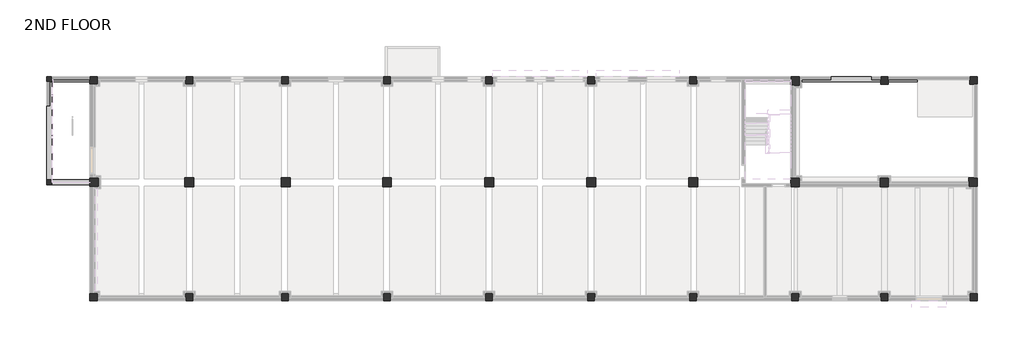
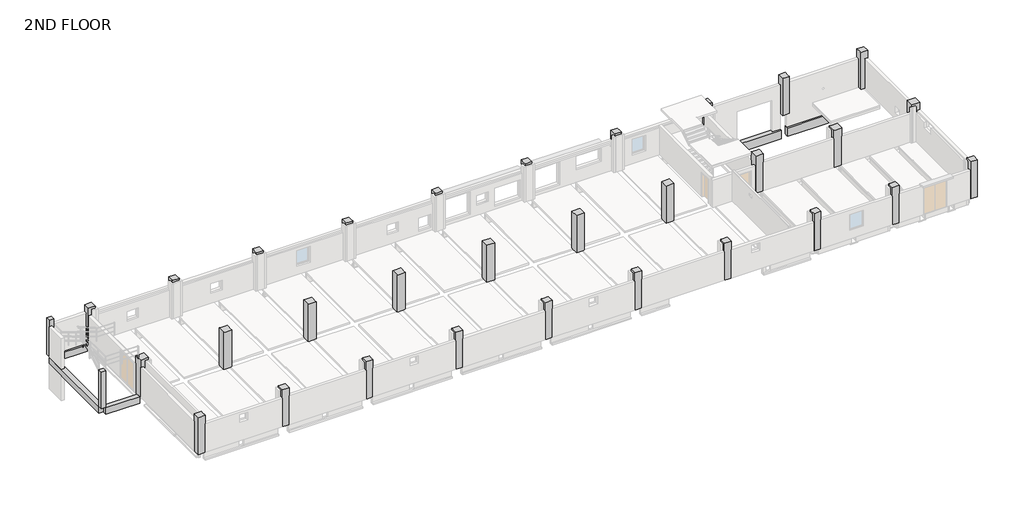
# One storey, part 5 of 7: 32 columns, 8 beams.
"""IFC4 building model written with IfcOpenShell, lengths in millimetres."""

from ifc_helpers import new_model, si_unit, frame, origin, place, context, project, spatial, polyline, outline, extrude, faceted_brep, element, save

model = new_model("IFC4")

# Units and contexts
model_context = context("Model", 3, world=origin())
ifc_project = project(units=[si_unit("LENGTHUNIT", "METRE", prefix="MILLI")], contexts=[model_context])

# Site, building, storey
site = spatial("IfcSite", under=ifc_project)
building = spatial("IfcBuilding", under=site)
storey = spatial("IfcBuildingStorey", under=building, Name="2ND FLOOR", Elevation=10600.0)

# Beams
placement = place(None, origin())
element("IfcBeam", 1, ObjectType="RC Beam_Rectangular : H_SB_AR S16_RC Beam-AG_400x800_2WG1", at=placement, inside=storey, context=model_context, shape_type="Brep", body=[
    faceted_brep([(61700.0, -100.0, 9100.0), (61700.0, 50.0, 9100.0), (61700.0, 300.0, 9100.0), (61000.0, 300.0, 9100.0), (57800.0, 300.0, 9100.0), (55350.0, 300.0, 9100.0), (55350.0, 50.0, 9100.0), (55350.0, -100.0, 9100.0), (61700.0, -100.0, 8300.0), (55350.0, -100.0, 8300.0), (61700.0, 300.0, 8300.0), (61700.0, 50.0, 8300.0), (55350.0, 50.0, 8300.0), (55350.0, 300.0, 8300.0)], [[[0, 1, 2, 3, 4, 5, 6, 7]], [[8, 0, 7, 9]], [[10, 11, 8, 9, 12, 13]], [[2, 10, 13, 5, 4, 3]], [[5, 13, 12, 9, 7, 6]], [[2, 1, 0, 8, 11, 10]]]),
])
element("IfcBeam", 2, ObjectType="RC Beam_Rectangular : H_SB_AR S16_RC Beam-AG_400x800_2WG1", at=placement, inside=storey, context=model_context, shape_type="Brep", body=[
    faceted_brep([(68700.0, -100.0, 9100.0), (68700.0, 50.0, 9100.0), (68700.0, 300.0, 9100.0), (62300.0, 300.0, 9100.0), (62300.0, 50.0, 9100.0), (62300.0, -100.0, 9100.0), (64775.0, -100.0, 9100.0), (64793.0, -100.0, 9100.0), (68700.0, -100.0, 8300.0), (62300.0, -100.0, 8300.0), (64775.0, -100.0, 8300.0), (64793.0, -100.0, 8300.0), (68700.0, 300.0, 8300.0), (68700.0, 50.0, 8300.0), (62300.0, 50.0, 8300.0), (62300.0, 300.0, 8300.0)], [[[0, 1, 2, 3, 4, 5, 6, 7]], [[8, 0, 7, 6, 5, 9, 10, 11]], [[12, 13, 8, 11, 10, 9, 14, 15]], [[2, 12, 15, 3]], [[3, 15, 14, 9, 5, 4]], [[2, 1, 0, 8, 13, 12]]]),
])
element("IfcBeam", 3, ObjectType="RC Beam_Rectangular : H_SB_AR S16_RC Beam-AG_400x600_SWG1", at=placement, inside=storey, context=model_context, shape_type="Brep", body=[
    faceted_brep([(-300.0, -100.0, 10550.0), (-300.0, 50.0, 10550.0), (-300.0, 300.0, 10550.0), (-3300.0, 300.0, 10550.0), (-3300.0, 50.0, 10550.0), (-3300.0, -100.0, 10550.0), (-300.0, -100.0, 9950.0), (-3300.0, -100.0, 9950.0), (-300.0, 300.0, 9950.0), (-300.0, 50.0, 9950.0), (-3300.0, 50.0, 9950.0), (-3300.0, 300.0, 9950.0)], [[[0, 1, 2, 3, 4, 5]], [[6, 0, 5, 7]], [[8, 9, 6, 7, 10, 11]], [[2, 8, 11, 3]], [[2, 1, 0, 6, 9, 8]], [[3, 11, 10, 7, 5, 4]]]),
])
element("IfcBeam", 4, ObjectType="RC Beam_Rectangular : H_SB_AR S16_RC Beam-AG_400x600_SWG2", at=placement, inside=storey, context=model_context, shape_type="Brep", body=[
    faceted_brep([(-3300.0, -100.0, 10550.0), (-3450.0, -100.0, 10550.0), (-3700.0, -100.0, 10550.0), (-3700.0, -2000.0, 10550.0), (-3700.0, -7800.0, 10550.0), (-3300.0, -7800.0, 10550.0), (-3300.0, -100.0, 9950.0), (-3300.0, -7800.0, 9950.0), (-3700.0, -100.0, 9950.0), (-3450.0, -100.0, 9950.0), (-3700.0, -7800.0, 9950.0), (-3700.0, -2000.0, 9950.0)], [[[0, 1, 2, 3, 4, 5]], [[6, 0, 5, 7]], [[8, 9, 6, 7, 10, 11]], [[2, 8, 11, 10, 4, 3]], [[4, 10, 7, 5]], [[2, 1, 0, 6, 9, 8]]]),
])
element("IfcBeam", 5, ObjectType="RC Beam_Rectangular : H_SB_AR S16_RC Beam-AG_400x600_SG1", at=placement, inside=storey, context=model_context, shape_type="SweptSolid", body=[
    extrude(outline(polyline([(-300.0, -7800.0), (-300.0, -8200.0), (-3300.0, -8200.0), (-3300.0, -7800.0), (-300.0, -7800.0)])), frame((0.0, 0.0, 9950.0), z_axis=(0.0, 0.0, 1.0), x_axis=(1.0, 0.0, 0.0)), (0.0, 0.0, 1.0), 600.0),
])
element("IfcBeam", 6, ObjectType="RC Beam_Rectangular : H_SB_AR S16_RC Beam-AG_300x500_2CB1", at=placement, inside=storey, context=model_context, shape_type="Brep", body=[
    faceted_brep([(22850.0, 300.0, 9300.0), (23000.0, 300.0, 9300.0), (23150.0, 300.0, 9300.0), (23150.0, 2350.0, 9300.0), (22850.0, 2350.0, 9300.0), (22850.0, 300.0, 8800.0), (22850.0, 2350.0, 8800.0), (23150.0, 300.0, 8800.0), (23150.0, 2350.0, 8800.0), (23150.0, 300.0, 9150.0), (23150.0, 2350.0, 9150.0)], [[[0, 1, 2, 3, 4]], [[5, 0, 4, 6]], [[7, 5, 6, 8]], [[2, 9, 7, 8, 10, 3]], [[2, 1, 0, 5, 7, 9]], [[3, 10, 8, 6, 4]]]),
])
element("IfcBeam", 7, ObjectType="RC Beam_Rectangular : H_SB_AR S16_RC Beam-AG_300x500_2CB1", at=placement, inside=storey, context=model_context, shape_type="Brep", body=[
    faceted_brep([(27150.0, 2350.0, 9300.0), (26850.0, 2350.0, 9300.0), (26850.0, 300.0, 9300.0), (27000.0, 300.0, 9300.0), (27150.0, 300.0, 9300.0), (26850.0, 2350.0, 9150.0), (26850.0, 2350.0, 8800.0), (26850.0, 300.0, 8800.0), (26850.0, 300.0, 9150.0), (27150.0, 2350.0, 8800.0), (27150.0, 300.0, 8800.0)], [[[0, 1, 2, 3, 4]], [[1, 5, 6, 7, 8, 2]], [[6, 9, 10, 7]], [[9, 0, 4, 10]], [[4, 3, 2, 8, 7, 10]], [[0, 9, 6, 5, 1]]]),
])
element("IfcBeam", 8, ObjectType="RC Beam_Rectangular : H_SB_AR S16_RC Beam-AG_300x500_2CB2", at=placement, inside=storey, context=model_context, shape_type="Brep", body=[
    faceted_brep([(26850.0, 2350.0, 9300.0), (26850.0, 2650.0, 9300.0), (23150.0, 2650.0, 9300.0), (23150.0, 2350.0, 9300.0), (26850.0, 2350.0, 8800.0), (26850.0, 2350.0, 9150.0), (23150.0, 2350.0, 9150.0), (23150.0, 2350.0, 8800.0), (26850.0, 2650.0, 8800.0), (23150.0, 2650.0, 8800.0)], [[[0, 1, 2, 3]], [[4, 5, 0, 3, 6, 7]], [[8, 4, 7, 9]], [[1, 8, 9, 2]], [[2, 9, 7, 6, 3]], [[1, 0, 5, 4, 8]]]),
])

# Columns
element("IfcColumn", 9, ObjectType="RC_Column_Rectangular : H_SC_AR S15_RC Col-AG_700x700_C1", at=placement, inside=storey, context=model_context, shape_type="Brep", body=[
    faceted_brep([(400.0, -7650.0, 10600.0), (400.0, -7700.0, 10600.0), (400.0, -8300.0, 10600.0), (400.0, -8350.0, 10600.0), (399.4974747, -8350.0, 10600.0), (-50.0, -8350.0, 10600.0), (-300.0, -8350.0, 10600.0), (-300.0, -7650.0, 10600.0), (-50.0, -7650.0, 10600.0), (399.4974747, -7650.0, 10600.0), (400.0, -7650.0, 13920.0), (400.0, -7700.0, 13920.0), (400.0, -7700.0, 14100.0), (400.0, -8300.0, 14100.0), (400.0, -8300.0, 13920.0), (400.0, -8350.0, 13920.0), (399.4974747, -8350.0, 13920.0), (399.4974747, -8350.0, 14100.0), (100.0, -8350.0, 14100.0), (-300.0, -8350.0, 14100.0), (-300.0, -8350.0, 13400.0), (-300.0, -7650.0, 14100.0), (-300.0, -7650.0, 13400.0), (100.0, -7650.0, 14100.0), (399.4974747, -7650.0, 14100.0), (399.4974747, -7650.0, 13920.0), (399.4974747, -8300.0, 14100.0), (399.4974747, -7700.0, 14100.0), (399.4974747, -7700.0, 13920.0), (399.4974747, -8300.0, 13920.0)], [[[0, 1, 2, 3, 4, 5, 6, 7, 8, 9]], [[3, 2, 1, 0, 10, 11, 12, 13, 14, 15]], [[6, 5, 4, 3, 15, 16, 17, 18, 19, 20]], [[7, 6, 20, 19, 21, 22]], [[0, 9, 8, 7, 22, 21, 23, 24, 25, 10]], [[21, 19, 18, 17, 26, 13, 12, 27, 24, 23]], [[25, 28, 11, 10]], [[28, 27, 12, 11]], [[28, 25, 24, 27]], [[16, 29, 26, 17]], [[26, 29, 14, 13]], [[29, 16, 15, 14]]]),
])
element("IfcColumn", 10, ObjectType="RC_Column_Rectangular : H_SC_AR S15_RC Col-AG_700x700_C1", at=placement, inside=storey, context=model_context, shape_type="Brep", body=[
    faceted_brep([(7850.0, -7650.0, 10600.0), (7850.0, -8350.0, 10600.0), (7150.0, -8350.0, 10600.0), (7150.0, -7650.0, 10600.0), (7850.0, -7650.0, 13920.0), (7850.0, -7650.0, 14100.0), (7850.0, -7700.0, 14100.0), (7850.0, -8300.0, 14100.0), (7850.0, -8350.0, 14100.0), (7850.0, -8350.0, 13920.0), (7750.0, -8350.0, 14100.0), (7250.0, -8350.0, 14100.0), (7150.0, -8350.0, 14100.0), (7150.0, -8350.0, 13920.0), (7150.0, -8300.0, 14100.0), (7150.0, -7700.0, 14100.0), (7150.0, -7650.0, 14100.0), (7150.0, -7650.0, 13920.0), (7250.0, -7650.0, 14100.0), (7750.0, -7650.0, 14100.0)], [[[0, 1, 2, 3]], [[1, 0, 4, 5, 6, 7, 8, 9]], [[2, 1, 9, 8, 10, 11, 12, 13]], [[3, 2, 13, 12, 14, 15, 16, 17]], [[0, 3, 17, 16, 18, 19, 5, 4]], [[18, 16, 15, 14, 12, 11, 10, 8, 7, 6, 5, 19]]]),
])
element("IfcColumn", 11, ObjectType="RC_Column_Rectangular : H_SC_AR S15_RC Col-AG_700x700_C1", at=placement, inside=storey, context=model_context, shape_type="Brep", body=[
    faceted_brep([(15400.0000001, -7650.0, 10600.0), (15400.0000001, -8350.0, 10600.0), (14700.0000001, -8350.0, 10600.0), (14700.0000001, -7650.0, 10600.0), (15400.0000001, -7650.0, 13920.0), (15400.0000001, -7650.0, 14100.0), (15400.0000001, -7700.0, 14100.0), (15400.0000001, -8300.0, 14100.0), (15400.0000001, -8350.0, 14100.0), (15400.0000001, -8350.0, 13920.0), (15250.0, -8350.0, 14100.0), (14750.0, -8350.0, 14100.0), (14700.0000001, -8350.0, 14100.0), (14700.0000001, -8350.0, 13920.0), (14700.0000001, -8300.0, 14100.0), (14700.0000001, -7700.0, 14100.0), (14700.0000001, -7650.0, 14100.0), (14700.0000001, -7650.0, 13920.0), (14750.0, -7650.0, 14100.0), (15250.0, -7650.0, 14100.0)], [[[0, 1, 2, 3]], [[1, 0, 4, 5, 6, 7, 8, 9]], [[2, 1, 9, 8, 10, 11, 12, 13]], [[3, 2, 13, 12, 14, 15, 16, 17]], [[0, 3, 17, 16, 18, 19, 5, 4]], [[5, 19, 18, 16, 15, 14, 12, 11, 10, 8, 7, 6]]]),
])
element("IfcColumn", 12, ObjectType="RC_Column_Rectangular : H_SC_AR S15_RC Col-AG_700x700_C1", at=placement, inside=storey, context=model_context, shape_type="Brep", body=[
    faceted_brep([(23350.0000003, -7650.0, 10600.0), (23350.0000003, -8350.0, 10600.0), (22650.0000003, -8350.0, 10600.0), (22650.0000003, -7650.0, 10600.0), (23350.0000003, -7650.0, 13920.0), (23350.0000003, -7650.0, 14100.0), (23350.0000003, -7700.0, 14100.0), (23350.0000003, -8300.0, 14100.0), (23350.0000003, -8350.0, 14100.0), (23350.0000003, -8350.0, 13920.0), (23250.0, -8350.0, 14100.0), (22750.0, -8350.0, 14100.0), (22650.0000003, -8350.0, 14100.0), (22650.0000003, -8350.0, 13920.0), (22650.0000003, -8300.0, 14100.0), (22650.0000003, -7700.0, 14100.0), (22650.0000003, -7650.0, 14100.0), (22650.0000003, -7650.0, 13920.0), (22750.0, -7650.0, 14100.0), (23250.0, -7650.0, 14100.0)], [[[0, 1, 2, 3]], [[1, 0, 4, 5, 6, 7, 8, 9]], [[2, 1, 9, 8, 10, 11, 12, 13]], [[3, 2, 13, 12, 14, 15, 16, 17]], [[0, 3, 17, 16, 18, 19, 5, 4]], [[18, 16, 15, 14, 12, 11, 10, 8, 7, 6, 5, 19]]]),
])
element("IfcColumn", 13, ObjectType="RC_Column_Rectangular : H_SC_AR S15_RC Col-AG_700x700_C1", at=placement, inside=storey, context=model_context, shape_type="Brep", body=[
    faceted_brep([(31350.0000002, -7650.0, 10600.0), (31350.0000002, -8350.0, 10600.0), (30650.0000002, -8350.0, 10600.0), (30650.0000002, -7650.0, 10600.0), (31350.0000002, -7650.0, 13920.0), (31350.0000002, -7650.0, 14100.0), (31350.0000002, -7700.0, 14100.0), (31350.0000002, -8300.0, 14100.0), (31350.0000002, -8350.0, 14100.0), (31350.0000002, -8350.0, 13920.0), (31249.9999998, -8350.0, 14100.0), (30750.0000002, -8350.0, 14100.0), (30650.0000002, -8350.0, 14100.0), (30650.0000002, -8350.0, 13920.0), (30650.0000002, -8300.0, 14100.0), (30650.0000002, -7700.0, 14100.0), (30650.0000002, -7650.0, 14100.0), (30650.0000002, -7650.0, 13920.0), (30750.0000002, -7650.0, 14100.0), (31249.9999998, -7650.0, 14100.0)], [[[0, 1, 2, 3]], [[1, 0, 4, 5, 6, 7, 8, 9]], [[2, 1, 9, 8, 10, 11, 12, 13]], [[3, 2, 13, 12, 14, 15, 16, 17]], [[0, 3, 17, 16, 18, 19, 5, 4]], [[18, 16, 15, 14, 12, 11, 10, 8, 7, 6, 5, 19]]]),
])
element("IfcColumn", 14, ObjectType="RC_Column_Rectangular : H_SC_AR S15_RC Col-AG_700x700_C1", at=placement, inside=storey, context=model_context, shape_type="Brep", body=[
    faceted_brep([(39350.0000001, -7650.0, 10600.0), (39350.0000001, -8350.0, 10600.0), (38650.0000001, -8350.0, 10600.0), (38650.0000001, -7650.0, 10600.0), (39350.0000001, -7650.0, 13920.0), (39350.0000001, -7650.0, 14100.0), (39350.0000001, -7700.0, 14100.0), (39350.0000001, -8300.0, 14100.0), (39350.0000001, -8350.0, 14100.0), (39350.0000001, -8350.0, 13920.0), (39249.9999998, -8350.0, 14100.0), (38750.0000002, -8350.0, 14100.0), (38650.0000001, -8350.0, 14100.0), (38650.0000001, -8350.0, 13920.0), (38650.0000001, -8300.0, 14100.0), (38650.0000001, -7700.0, 14100.0), (38650.0000001, -7650.0, 14100.0), (38650.0000001, -7650.0, 13920.0), (38750.0000002, -7650.0, 14100.0), (39249.9999998, -7650.0, 14100.0)], [[[0, 1, 2, 3]], [[1, 0, 4, 5, 6, 7, 8, 9]], [[2, 1, 9, 8, 10, 11, 12, 13]], [[3, 2, 13, 12, 14, 15, 16, 17]], [[0, 3, 17, 16, 18, 19, 5, 4]], [[18, 16, 15, 14, 12, 11, 10, 8, 7, 6, 5, 19]]]),
])
element("IfcColumn", 15, ObjectType="RC_Column_Rectangular : H_SC_AR S15_RC Col-AG_700x700_C1", at=placement, inside=storey, context=model_context, shape_type="Brep", body=[
    faceted_brep([(47349.9999999, -7650.0, 10600.0), (47349.9999999, -8350.0, 10600.0), (46649.9999999, -8350.0, 10600.0), (46649.9999999, -7650.0, 10600.0), (47349.9999999, -7650.0, 13920.0), (47349.9999999, -7650.0, 14100.0), (47349.9999999, -7750.0, 14100.0), (47349.9999999, -8350.0, 14100.0), (47349.9999999, -8350.0, 13920.0), (47250.0, -8350.0, 14100.0), (46750.0, -8350.0, 14100.0), (46649.9999999, -8350.0, 14100.0), (46649.9999999, -8350.0, 13920.0), (46649.9999999, -8300.0, 14100.0), (46649.9999999, -7700.0, 14100.0), (46649.9999999, -7650.0, 14100.0), (46649.9999999, -7650.0, 13920.0), (46750.0, -7650.0, 14100.0), (47250.0, -7650.0, 14100.0)], [[[0, 1, 2, 3]], [[1, 0, 4, 5, 6, 7, 8]], [[2, 1, 8, 7, 9, 10, 11, 12]], [[3, 2, 12, 11, 13, 14, 15, 16]], [[0, 3, 16, 15, 17, 18, 5, 4]], [[17, 15, 14, 13, 11, 10, 9, 7, 6, 5, 18]]]),
])
element("IfcColumn", 16, ObjectType="RC_Column_Rectangular : H_SC_AR S15_RC Col-AG_700x700_C1", at=placement, inside=storey, context=model_context, shape_type="Brep", body=[
    faceted_brep([(55350.0, -7650.0, 10600.0), (55350.0, -8100.0, 10600.0), (55350.0, -8350.0, 10600.0), (54650.0, -8350.0, 10600.0), (54650.0, -8100.0, 10600.0), (54650.0, -7650.0, 10600.0), (54900.0, -7650.0, 10600.0), (55350.0, -7650.0, 13920.0), (55350.0, -7650.0, 14100.0), (55350.0, -7750.0, 14100.0), (55350.0, -8350.0, 14100.0), (55350.0, -8350.0, 13920.0), (55350.0, -8350.0, 13300.0), (55200.0, -8350.0, 14100.0), (54700.0, -8350.0, 14100.0), (54650.0, -8350.0, 14100.0), (54650.0, -8350.0, 13920.0), (54650.0, -8350.0, 13200.0), (54650.0, -7650.0, 14100.0), (54650.0, -7650.0, 13300.0), (55150.0, -7650.0, 14100.0)], [[[0, 1, 2, 3, 4, 5, 6]], [[2, 1, 0, 7, 8, 9, 10, 11, 12]], [[3, 2, 12, 11, 10, 13, 14, 15, 16, 17]], [[5, 4, 3, 17, 16, 15, 18, 19]], [[0, 6, 5, 19, 18, 20, 8, 7]], [[18, 15, 14, 13, 10, 9, 8, 20]]]),
])
element("IfcColumn", 17, ObjectType="RC_Column_Rectangular : H_SC_AR S15_RC Col-AG_700x700_C1", at=placement, inside=storey, context=model_context, shape_type="Brep", body=[
    faceted_brep([(62350.0, -7650.0, 10600.0), (62350.0, -8100.0, 10600.0), (62350.0, -8350.0, 10600.0), (61650.0, -8350.0, 10600.0), (61650.0, -8100.0, 10600.0), (61650.0, -7650.0, 10600.0), (62350.0, -7650.0, 13920.0), (62350.0, -7650.0, 14100.0), (62350.0, -7750.0, 14100.0), (62350.0, -8350.0, 14100.0), (62350.0, -8350.0, 13920.0), (62350.0, -8350.0, 13300.0), (62250.0, -8350.0, 14100.0), (61750.0, -8350.0, 14100.0), (61650.0, -8350.0, 14100.0), (61650.0, -8350.0, 13920.0), (61650.0, -8350.0, 13300.0), (61650.0, -7750.0, 14100.0), (61650.0, -7650.0, 14100.0), (61650.0, -7650.0, 13920.0), (61750.0, -7650.0, 14100.0), (62250.0, -7650.0, 14100.0)], [[[0, 1, 2, 3, 4, 5]], [[2, 1, 0, 6, 7, 8, 9, 10, 11]], [[3, 2, 11, 10, 9, 12, 13, 14, 15, 16]], [[5, 4, 3, 16, 15, 14, 17, 18, 19]], [[0, 5, 19, 18, 20, 21, 7, 6]], [[20, 18, 17, 14, 13, 12, 9, 8, 7, 21]]]),
])
element("IfcColumn", 18, ObjectType="RC_Column_Rectangular : H_SC_AR S15_RC Col-AG_700x700_C1", at=placement, inside=storey, context=model_context, shape_type="Brep", body=[
    faceted_brep([(69300.0, -7650.0, 10600.0), (69300.0, -8350.0, 10600.0), (69050.0, -8350.0, 10600.0), (68600.0, -8350.0, 10600.0), (68600.0, -8100.0, 10600.0), (68600.0, -7650.0, 10600.0), (69050.0, -7650.0, 10600.0), (69300.0, -7650.0, 13400.0), (69300.0, -7650.0, 14100.0), (69300.0, -8350.0, 14100.0), (69300.0, -8350.0, 13400.0), (68900.0, -8350.0, 14100.0), (68600.0, -8350.0, 14100.0), (68600.0, -8350.0, 13920.0), (68600.0, -8350.0, 13300.0), (68600.0, -7750.0, 14100.0), (68600.0, -7650.0, 14100.0), (68600.0, -7650.0, 13920.0), (68900.0, -7650.0, 14100.0)], [[[0, 1, 2, 3, 4, 5, 6]], [[1, 0, 7, 8, 9, 10]], [[3, 2, 1, 10, 9, 11, 12, 13, 14]], [[5, 4, 3, 14, 13, 12, 15, 16, 17]], [[0, 6, 5, 17, 16, 18, 8, 7]], [[9, 8, 18, 16, 15, 12, 11]]]),
])
element("IfcColumn", 19, ObjectType="RC_Column_Rectangular : H_SC_AR S15_RC Col-AG_700x700_C1", at=placement, inside=storey, context=model_context, shape_type="Brep", body=[
    faceted_brep([(55350.0, 300.0, 10600.0), (55350.0, -400.0, 10600.0), (54900.0, -400.0, 10600.0), (54650.0, -400.0, 10600.0), (54650.0, 50.0, 10600.0), (54650.0, 300.0, 10600.0), (55350.0, 300.0, 13300.0), (55350.0, 300.0, 14100.0), (55350.0, -100.0, 14100.0), (55350.0, -400.0, 14100.0), (55350.0, -400.0, 13920.0), (55150.0, -400.0, 14100.0), (54900.0, -400.0, 14100.0), (54650.0, -400.0, 14100.0), (54650.0, -400.0, 13300.0), (54650.0, -387.0, 14100.0), (54650.0, 300.0, 14100.0), (54650.0, 300.0, 13300.0)], [[[0, 1, 2, 3, 4, 5]], [[1, 0, 6, 7, 8, 9, 10]], [[3, 2, 1, 10, 9, 11, 12, 13, 14]], [[5, 4, 3, 14, 13, 15, 16, 17]], [[0, 5, 17, 16, 7, 6]], [[16, 15, 13, 12, 11, 9, 8, 7]]]),
])
element("IfcColumn", 20, ObjectType="RC_Column_Rectangular : H_SC_AR S15_RC Col-AG_600x600_C2", at=placement, inside=storey, context=model_context, shape_type="Brep", body=[
    faceted_brep([(300.0, 300.0, 10600.0), (300.0, 50.0, 10600.0), (300.0, -300.0, 10600.0), (-50.0, -300.0, 10600.0), (-300.0, -300.0, 10600.0), (-300.0, 300.0, 10600.0), (300.0, 300.0, 13300.0), (300.0, 300.0, 14100.0), (300.0, -100.0, 14100.0), (300.0, -300.0, 14100.0), (300.0, -300.0, 13920.0), (100.0, -300.0, 14100.0), (-300.0, -300.0, 14100.0), (-300.0, -300.0, 13400.0), (-300.0, 300.0, 14100.0), (-300.0, 300.0, 14050.0), (-300.0, 300.0, 13450.0)], [[[0, 1, 2, 3, 4, 5]], [[2, 1, 0, 6, 7, 8, 9, 10]], [[4, 3, 2, 10, 9, 11, 12, 13]], [[5, 4, 13, 12, 14, 15, 16]], [[0, 5, 16, 15, 14, 7, 6]], [[14, 12, 11, 9, 8, 7]]]),
])
element("IfcColumn", 21, ObjectType="RC_Column_Rectangular : H_SC_AR S15_RC Col-AG_600x600_C2", at=placement, inside=storey, context=model_context, shape_type="Brep", body=[
    faceted_brep([(7800.0, 300.0, 10600.0), (7800.0, 50.0, 10600.0), (7800.0, -300.0, 10600.0), (7200.0, -300.0, 10600.0), (7200.0, 50.0, 10600.0), (7200.0, 300.0, 10600.0), (7800.0, 300.0, 13300.0), (7800.0, 300.0, 14100.0), (7800.0, -100.0, 14100.0), (7800.0, -300.0, 14100.0), (7800.0, -300.0, 13920.0), (7750.0, -300.0, 14100.0), (7250.0, -300.0, 14100.0), (7200.0, -300.0, 14100.0), (7200.0, -300.0, 13920.0), (7200.0, -100.0, 14100.0), (7200.0, 300.0, 14100.0), (7200.0, 300.0, 13300.0)], [[[0, 1, 2, 3, 4, 5]], [[2, 1, 0, 6, 7, 8, 9, 10]], [[3, 2, 10, 9, 11, 12, 13, 14]], [[5, 4, 3, 14, 13, 15, 16, 17]], [[0, 5, 17, 16, 7, 6]], [[7, 16, 15, 13, 12, 11, 9, 8]]]),
])
element("IfcColumn", 22, ObjectType="RC_Column_Rectangular : H_SC_AR S15_RC Col-AG_600x600_C2", at=placement, inside=storey, context=model_context, shape_type="Brep", body=[
    faceted_brep([(15300.0, 300.0, 10600.0), (15300.0, 50.0, 10600.0), (15300.0, -300.0, 10600.0), (14700.0, -300.0, 10600.0), (14700.0, 50.0, 10600.0), (14700.0, 300.0, 10600.0), (15300.0, 300.0, 13300.0), (15300.0, 300.0, 14100.0), (15300.0, -100.0, 14100.0), (15300.0, -300.0, 14100.0), (15300.0, -300.0, 13920.0), (15250.0, -300.0, 14100.0), (14750.0, -300.0, 14100.0), (14700.0, -300.0, 14100.0), (14700.0, -300.0, 13920.0), (14700.0, -100.0, 14100.0), (14700.0, 300.0, 14100.0), (14700.0, 300.0, 13300.0)], [[[0, 1, 2, 3, 4, 5]], [[2, 1, 0, 6, 7, 8, 9, 10]], [[3, 2, 10, 9, 11, 12, 13, 14]], [[5, 4, 3, 14, 13, 15, 16, 17]], [[0, 5, 17, 16, 7, 6]], [[7, 16, 15, 13, 12, 11, 9, 8]]]),
])
element("IfcColumn", 23, ObjectType="RC_Column_Rectangular : H_SC_AR S15_RC Col-AG_600x600_C2", at=placement, inside=storey, context=model_context, shape_type="Brep", body=[
    faceted_brep([(23300.0, 300.0, 10600.0), (23300.0, 50.0, 10600.0), (23300.0, -300.0, 10600.0), (22700.0, -300.0, 10600.0), (22700.0, 50.0, 10600.0), (22700.0, 300.0, 10600.0), (23300.0, 300.0, 13300.0), (23300.0, 300.0, 14100.0), (23300.0, -100.0, 14100.0), (23300.0, -300.0, 14100.0), (23300.0, -300.0, 13920.0), (23250.0, -300.0, 14100.0), (22750.0, -300.0, 14100.0), (22700.0, -300.0, 14100.0), (22700.0, -300.0, 13920.0), (22700.0, -100.0, 14100.0), (22700.0, 300.0, 14100.0), (22700.0, 300.0, 13300.0)], [[[0, 1, 2, 3, 4, 5]], [[2, 1, 0, 6, 7, 8, 9, 10]], [[3, 2, 10, 9, 11, 12, 13, 14]], [[5, 4, 3, 14, 13, 15, 16, 17]], [[0, 5, 17, 16, 7, 6]], [[7, 16, 15, 13, 12, 11, 9, 8]]]),
])
element("IfcColumn", 24, ObjectType="RC_Column_Rectangular : H_SC_AR S15_RC Col-AG_600x600_C2", at=placement, inside=storey, context=model_context, shape_type="Brep", body=[
    faceted_brep([(31300.0, 300.0, 10600.0), (31300.0, 50.0, 10600.0), (31300.0, -300.0, 10600.0), (30700.0, -300.0, 10600.0), (30700.0, 50.0, 10600.0), (30700.0, 300.0, 10600.0), (31300.0, 300.0, 13300.0), (31300.0, 300.0, 14100.0), (31300.0, -100.0, 14100.0), (31300.0, -300.0, 14100.0), (31300.0, -300.0, 13920.0), (31249.9999998, -300.0, 14100.0), (30750.0000002, -300.0, 14100.0), (30700.0, -300.0, 14100.0), (30700.0, -300.0, 13920.0), (30700.0, -100.0, 14100.0), (30700.0, 300.0, 14100.0), (30700.0, 300.0, 13300.0)], [[[0, 1, 2, 3, 4, 5]], [[2, 1, 0, 6, 7, 8, 9, 10]], [[3, 2, 10, 9, 11, 12, 13, 14]], [[5, 4, 3, 14, 13, 15, 16, 17]], [[0, 5, 17, 16, 7, 6]], [[7, 16, 15, 13, 12, 11, 9, 8]]]),
])
element("IfcColumn", 25, ObjectType="RC_Column_Rectangular : H_SC_AR S15_RC Col-AG_600x600_C2", at=placement, inside=storey, context=model_context, shape_type="Brep", body=[
    faceted_brep([(39300.0, 300.0, 10600.0), (39300.0, 50.0, 10600.0), (39300.0, -300.0, 10600.0), (38700.0, -300.0, 10600.0), (38700.0, 50.0, 10600.0), (38700.0, 300.0, 10600.0), (39300.0, 300.0, 13300.0), (39300.0, 300.0, 14100.0), (39300.0, -100.0, 14100.0), (39300.0, -300.0, 14100.0), (39300.0, -300.0, 13920.0), (39249.9999998, -300.0, 14100.0), (38750.0000002, -300.0, 14100.0), (38700.0, -300.0, 14100.0), (38700.0, -300.0, 13920.0), (38700.0, -100.0, 14100.0), (38700.0, 300.0, 14100.0), (38700.0, 300.0, 13300.0)], [[[0, 1, 2, 3, 4, 5]], [[2, 1, 0, 6, 7, 8, 9, 10]], [[3, 2, 10, 9, 11, 12, 13, 14]], [[5, 4, 3, 14, 13, 15, 16, 17]], [[0, 5, 17, 16, 7, 6]], [[7, 16, 15, 13, 12, 11, 9, 8]]]),
])
element("IfcColumn", 26, ObjectType="RC_Column_Rectangular : H_SC_AR S15_RC Col-AG_600x600_C2", at=placement, inside=storey, context=model_context, shape_type="Brep", body=[
    faceted_brep([(47300.0, 300.0, 10600.0), (47300.0, 50.0, 10600.0), (47300.0, -300.0, 10600.0), (46700.0, -300.0, 10600.0), (46700.0, 50.0, 10600.0), (46700.0, 300.0, 10600.0), (47300.0, 300.0, 13300.0), (47300.0, 300.0, 14100.0), (47300.0, -100.0, 14100.0), (47300.0, -300.0, 14100.0), (47300.0, -300.0, 13920.0), (47250.0, -300.0, 14100.0), (46750.0, -300.0, 14100.0), (46700.0, -300.0, 14100.0), (46700.0, -300.0, 13920.0), (46700.0, -100.0, 14100.0), (46700.0, 300.0, 14100.0), (46700.0, 300.0, 13300.0)], [[[0, 1, 2, 3, 4, 5]], [[2, 1, 0, 6, 7, 8, 9, 10]], [[3, 2, 10, 9, 11, 12, 13, 14]], [[5, 4, 3, 14, 13, 15, 16, 17]], [[0, 5, 17, 16, 7, 6]], [[7, 16, 15, 13, 12, 11, 9, 8]]]),
])
element("IfcColumn", 27, ObjectType="RC_Column_Rectangular : H_SC_AR S15_RC Col-AG_600x600_C2", at=placement, inside=storey, context=model_context, shape_type="Brep", body=[
    faceted_brep([(62300.0, 300.0, 10600.0), (62300.0, -300.0, 10600.0), (61700.0, -300.0, 10600.0), (61700.0, 300.0, 10600.0), (62300.0, 300.0, 13300.0), (62300.0, 300.0, 14100.0), (62300.0, -100.0, 14100.0), (62300.0, -300.0, 14100.0), (62300.0, -300.0, 13920.0), (62250.0, -300.0, 14100.0), (61750.0, -300.0, 14100.0), (61700.0, -300.0, 14100.0), (61700.0, -300.0, 13920.0), (61700.0, -100.0, 14100.0), (61700.0, 300.0, 14100.0), (61700.0, 300.0, 13300.0)], [[[0, 1, 2, 3]], [[1, 0, 4, 5, 6, 7, 8]], [[2, 1, 8, 7, 9, 10, 11, 12]], [[3, 2, 12, 11, 13, 14, 15]], [[0, 3, 15, 14, 5, 4]], [[5, 14, 13, 11, 10, 9, 7, 6]]]),
])
element("IfcColumn", 28, ObjectType="RC_Column_Rectangular : H_SC_AR S15_RC Col-AG_600x600_C2", at=placement, inside=storey, context=model_context, shape_type="Brep", body=[
    faceted_brep([(69300.0, 300.0, 10600.0), (69300.0, -300.0, 10600.0), (69050.0, -300.0, 10600.0), (68700.0, -300.0, 10600.0), (68700.0, 300.0, 10600.0), (69300.0, 300.0, 14100.0), (69300.0, -300.0, 14100.0), (69300.0, -300.0, 13400.0), (68900.0, -300.0, 14100.0), (68700.0, -300.0, 14100.0), (68700.0, -300.0, 13920.0), (68700.0, -100.0, 14100.0), (68700.0, 300.0, 14100.0), (68700.0, 300.0, 13300.0)], [[[0, 1, 2, 3, 4]], [[1, 0, 5, 6, 7]], [[3, 2, 1, 7, 6, 8, 9, 10]], [[4, 3, 10, 9, 11, 12, 13]], [[0, 4, 13, 12, 5]], [[6, 5, 12, 11, 9, 8]]]),
])
element("IfcColumn", 29, ObjectType="RC_Column_Rectangular : H_SC_AR S15_RC Col-AG_600x600_C2", at=placement, inside=storey, context=model_context, shape_type="Brep", body=[
    faceted_brep([(69300.0, -16700.0, 10600.0), (69300.0, -17300.0, 10600.0), (68700.0, -17300.0, 10600.0), (68700.0, -17050.0, 10600.0), (68700.0, -16700.0, 10600.0), (69050.0, -16700.0, 10600.0), (69300.0, -16700.0, 13400.0), (69300.0, -16700.0, 14100.0), (69300.0, -17300.0, 14100.0), (68700.0, -17300.0, 14100.0), (68700.0, -17300.0, 13300.0), (68700.0, -16900.0, 14100.0), (68700.0, -16700.0, 14100.0), (68700.0, -16700.0, 13920.0), (68900.0, -16700.0, 14100.0)], [[[0, 1, 2, 3, 4, 5]], [[1, 0, 6, 7, 8]], [[2, 1, 8, 9, 10]], [[4, 3, 2, 10, 9, 11, 12, 13]], [[0, 5, 4, 13, 12, 14, 7, 6]], [[8, 7, 14, 12, 11, 9]]]),
])
element("IfcColumn", 30, ObjectType="RC_Column_Rectangular : H_SC_AR S15_RC Col-AG_600x600_C2", at=placement, inside=storey, context=model_context, shape_type="Brep", body=[
    faceted_brep([(62300.0, -16700.0, 10600.0), (62300.0, -17050.0, 10600.0), (62300.0, -17300.0, 10600.0), (61700.0, -17300.0, 10600.0), (61700.0, -17050.0, 10600.0), (61700.0, -16700.0, 10600.0), (62300.0, -16700.0, 13920.0), (62300.0, -16700.0, 14100.0), (62300.0, -16900.0, 14100.0), (62300.0, -17300.0, 14100.0), (62300.0, -17300.0, 13300.0), (61700.0, -17300.0, 14100.0), (61700.0, -17300.0, 13300.0), (61700.0, -16900.0, 14100.0), (61700.0, -16700.0, 14100.0), (61700.0, -16700.0, 13920.0), (61750.0, -16700.0, 14100.0), (62250.0, -16700.0, 14100.0)], [[[0, 1, 2, 3, 4, 5]], [[2, 1, 0, 6, 7, 8, 9, 10]], [[3, 2, 10, 9, 11, 12]], [[5, 4, 3, 12, 11, 13, 14, 15]], [[0, 5, 15, 14, 16, 17, 7, 6]], [[11, 9, 8, 7, 17, 16, 14, 13]]]),
])
element("IfcColumn", 31, ObjectType="RC_Column_Rectangular : H_SC_AR S15_RC Col-AG_600x600_C2", at=placement, inside=storey, context=model_context, shape_type="Brep", body=[
    faceted_brep([(55300.0, -16700.0, 10600.0), (55300.0, -17050.0, 10600.0), (55300.0, -17300.0, 10600.0), (54700.0, -17300.0, 10600.0), (54700.0, -17050.0, 10600.0), (54700.0, -16700.0, 10600.0), (55300.0, -16700.0, 13920.0), (55300.0, -16700.0, 14100.0), (55300.0, -16900.0, 14100.0), (55300.0, -17300.0, 14100.0), (55300.0, -17300.0, 13300.0), (54700.0, -17300.0, 14100.0), (54700.0, -17300.0, 13300.0), (54700.0, -16900.0, 14100.0), (54700.0, -16700.0, 14100.0), (54700.0, -16700.0, 13920.0), (55200.0, -16700.0, 14100.0)], [[[0, 1, 2, 3, 4, 5]], [[2, 1, 0, 6, 7, 8, 9, 10]], [[3, 2, 10, 9, 11, 12]], [[5, 4, 3, 12, 11, 13, 14, 15]], [[0, 5, 15, 14, 16, 7, 6]], [[11, 9, 8, 7, 16, 14, 13]]]),
])
element("IfcColumn", 32, ObjectType="RC_Column_Rectangular : H_SC_AR S15_RC Col-AG_600x600_C2", at=placement, inside=storey, context=model_context, shape_type="Brep", body=[
    faceted_brep([(46700.0, -16700.0, 10600.0), (47300.0, -16700.0, 10600.0), (47300.0, -17050.0, 10600.0), (47300.0, -17300.0, 10600.0), (46700.0, -17300.0, 10600.0), (46700.0, -17050.0, 10600.0), (46700.0, -16700.0, 13920.0), (46700.0, -16700.0, 14100.0), (46750.0, -16700.0, 14100.0), (47250.0, -16700.0, 14100.0), (47300.0, -16700.0, 14100.0), (47300.0, -16700.0, 13920.0), (47300.0, -16900.0, 14100.0), (47300.0, -17300.0, 14100.0), (47300.0, -17300.0, 13300.0), (46700.0, -17300.0, 14100.0), (46700.0, -17300.0, 13300.0), (46700.0, -16900.0, 14100.0)], [[[0, 1, 2, 3, 4, 5]], [[1, 0, 6, 7, 8, 9, 10, 11]], [[3, 2, 1, 11, 10, 12, 13, 14]], [[4, 3, 14, 13, 15, 16]], [[0, 5, 4, 16, 15, 17, 7, 6]], [[15, 13, 12, 10, 9, 8, 7, 17]]]),
])
element("IfcColumn", 33, ObjectType="RC_Column_Rectangular : H_SC_AR S15_RC Col-AG_600x600_C2", at=placement, inside=storey, context=model_context, shape_type="Brep", body=[
    faceted_brep([(38700.0, -16700.0, 10600.0), (39300.0, -16700.0, 10600.0), (39300.0, -17050.0, 10600.0), (39300.0, -17300.0, 10600.0), (38700.0, -17300.0, 10600.0), (38700.0, -17050.0, 10600.0), (38700.0, -16700.0, 13920.0), (38700.0, -16700.0, 14100.0), (38750.0000002, -16700.0, 14100.0), (39249.9999998, -16700.0, 14100.0), (39300.0, -16700.0, 14100.0), (39300.0, -16700.0, 13920.0), (39300.0, -16900.0, 14100.0), (39300.0, -17300.0, 14100.0), (39300.0, -17300.0, 13300.0), (38700.0, -17300.0, 14100.0), (38700.0, -17300.0, 13300.0), (38700.0, -16900.0, 14100.0)], [[[0, 1, 2, 3, 4, 5]], [[1, 0, 6, 7, 8, 9, 10, 11]], [[3, 2, 1, 11, 10, 12, 13, 14]], [[4, 3, 14, 13, 15, 16]], [[0, 5, 4, 16, 15, 17, 7, 6]], [[15, 13, 12, 10, 9, 8, 7, 17]]]),
])
element("IfcColumn", 34, ObjectType="RC_Column_Rectangular : H_SC_AR S15_RC Col-AG_600x600_C2", at=placement, inside=storey, context=model_context, shape_type="Brep", body=[
    faceted_brep([(30700.0, -16700.0, 10600.0), (31300.0, -16700.0, 10600.0), (31300.0, -17050.0, 10600.0), (31300.0, -17300.0, 10600.0), (30700.0, -17300.0, 10600.0), (30700.0, -17050.0, 10600.0), (30700.0, -16700.0, 13920.0), (30700.0, -16700.0, 14100.0), (30750.0000002, -16700.0, 14100.0), (31249.9999998, -16700.0, 14100.0), (31300.0, -16700.0, 14100.0), (31300.0, -16700.0, 13920.0), (31300.0, -16900.0, 14100.0), (31300.0, -17300.0, 14100.0), (31300.0, -17300.0, 13300.0), (30700.0, -17300.0, 14100.0), (30700.0, -17300.0, 13300.0), (30700.0, -16900.0, 14100.0)], [[[0, 1, 2, 3, 4, 5]], [[1, 0, 6, 7, 8, 9, 10, 11]], [[3, 2, 1, 11, 10, 12, 13, 14]], [[4, 3, 14, 13, 15, 16]], [[0, 5, 4, 16, 15, 17, 7, 6]], [[15, 13, 12, 10, 9, 8, 7, 17]]]),
])
element("IfcColumn", 35, ObjectType="RC_Column_Rectangular : H_SC_AR S15_RC Col-AG_600x600_C2", at=placement, inside=storey, context=model_context, shape_type="Brep", body=[
    faceted_brep([(22700.0, -16700.0, 10600.0), (23300.0, -16700.0, 10600.0), (23300.0, -17050.0, 10600.0), (23300.0, -17300.0, 10600.0), (22700.0, -17300.0, 10600.0), (22700.0, -17050.0, 10600.0), (22700.0, -16700.0, 13920.0), (22700.0, -16700.0, 14100.0), (22750.0, -16700.0, 14100.0), (23250.0, -16700.0, 14100.0), (23300.0, -16700.0, 14100.0), (23300.0, -16700.0, 13920.0), (23300.0, -16900.0, 14100.0), (23300.0, -17300.0, 14100.0), (23300.0, -17300.0, 13300.0), (22700.0, -17300.0, 14100.0), (22700.0, -17300.0, 13300.0), (22700.0, -16900.0, 14100.0)], [[[0, 1, 2, 3, 4, 5]], [[1, 0, 6, 7, 8, 9, 10, 11]], [[3, 2, 1, 11, 10, 12, 13, 14]], [[4, 3, 14, 13, 15, 16]], [[0, 5, 4, 16, 15, 17, 7, 6]], [[15, 13, 12, 10, 9, 8, 7, 17]]]),
])
element("IfcColumn", 36, ObjectType="RC_Column_Rectangular : H_SC_AR S15_RC Col-AG_600x600_C2", at=placement, inside=storey, context=model_context, shape_type="Brep", body=[
    faceted_brep([(14700.0, -16700.0, 10600.0), (15300.0, -16700.0, 10600.0), (15300.0, -17050.0, 10600.0), (15300.0, -17300.0, 10600.0), (14700.0, -17300.0, 10600.0), (14700.0, -17050.0, 10600.0), (14700.0, -16700.0, 13920.0), (14700.0, -16700.0, 14100.0), (14750.0, -16700.0, 14100.0), (15250.0, -16700.0, 14100.0), (15300.0, -16700.0, 14100.0), (15300.0, -16700.0, 13920.0), (15300.0, -16900.0, 14100.0), (15300.0, -17300.0, 14100.0), (15300.0, -17300.0, 13300.0), (14700.0, -17300.0, 14100.0), (14700.0, -17300.0, 13300.0), (14700.0, -16900.0, 14100.0)], [[[0, 1, 2, 3, 4, 5]], [[1, 0, 6, 7, 8, 9, 10, 11]], [[3, 2, 1, 11, 10, 12, 13, 14]], [[4, 3, 14, 13, 15, 16]], [[0, 5, 4, 16, 15, 17, 7, 6]], [[15, 13, 12, 10, 9, 8, 7, 17]]]),
])
element("IfcColumn", 37, ObjectType="RC_Column_Rectangular : H_SC_AR S15_RC Col-AG_600x600_C2", at=placement, inside=storey, context=model_context, shape_type="Brep", body=[
    faceted_brep([(7200.0, -16700.0, 10600.0), (7800.0, -16700.0, 10600.0), (7800.0, -17050.0, 10600.0), (7800.0, -17300.0, 10600.0), (7200.0, -17300.0, 10600.0), (7200.0, -17050.0, 10600.0), (7200.0, -16700.0, 13920.0), (7200.0, -16700.0, 14100.0), (7250.0, -16700.0, 14100.0), (7750.0, -16700.0, 14100.0), (7800.0, -16700.0, 14100.0), (7800.0, -16700.0, 13920.0), (7800.0, -16900.0, 14100.0), (7800.0, -17300.0, 14100.0), (7800.0, -17300.0, 13300.0), (7200.0, -17300.0, 14100.0), (7200.0, -17300.0, 13300.0), (7200.0, -16900.0, 14100.0)], [[[0, 1, 2, 3, 4, 5]], [[1, 0, 6, 7, 8, 9, 10, 11]], [[3, 2, 1, 11, 10, 12, 13, 14]], [[4, 3, 14, 13, 15, 16]], [[0, 5, 4, 16, 15, 17, 7, 6]], [[15, 13, 12, 10, 9, 8, 7, 17]]]),
])
element("IfcColumn", 38, ObjectType="RC_Column_Rectangular : H_SC_AR S15_RC Col-AG_600x600_C2", at=placement, inside=storey, context=model_context, shape_type="Brep", body=[
    faceted_brep([(-300.0, -16700.0, 10600.0), (-50.0, -16700.0, 10600.0), (300.0, -16700.0, 10600.0), (300.0, -17050.0, 10600.0), (300.0, -17300.0, 10600.0), (-300.0, -17300.0, 10600.0), (-300.0, -16700.0, 13400.0), (-300.0, -16700.0, 14100.0), (100.0, -16700.0, 14100.0), (300.0, -16700.0, 14100.0), (300.0, -16700.0, 13920.0), (300.0, -16900.0, 14100.0), (300.0, -17300.0, 14100.0), (300.0, -17300.0, 13300.0), (-300.0, -17300.0, 14100.0)], [[[0, 1, 2, 3, 4, 5]], [[2, 1, 0, 6, 7, 8, 9, 10]], [[4, 3, 2, 10, 9, 11, 12, 13]], [[5, 4, 13, 12, 14]], [[0, 5, 14, 7, 6]], [[14, 12, 11, 9, 8, 7]]]),
])
element("IfcColumn", 39, ObjectType="RC_Column_Rectangular : H_SC_AR S15_RC Col-AG_400x400_C3", at=placement, inside=storey, context=model_context, shape_type="Brep", body=[
    faceted_brep([(-3300.0, -7800.0, 10600.0), (-3300.0, -8200.0, 10600.0), (-3700.0, -8200.0, 10600.0), (-3700.0, -7800.0, 10600.0), (-3300.0, -7800.0, 14050.0), (-3300.0, -8200.0, 14050.0), (-3300.0, -7800.0, 13450.0), (-3700.0, -8200.0, 14050.0), (-3700.0, -7800.0, 14050.0), (-3700.0, -7800.0, 13450.0)], [[[0, 1, 2, 3]], [[4, 5, 1, 0, 6]], [[5, 7, 2, 1]], [[7, 8, 9, 3, 2]], [[8, 4, 6, 0, 3, 9]], [[4, 8, 7, 5]]]),
])
element("IfcColumn", 40, ObjectType="RC_Column_Rectangular : H_SC_AR S15_RC Col-AG_400x400_C3", at=placement, inside=storey, context=model_context, shape_type="Brep", body=[
    faceted_brep([(-3300.0, 300.0, 10600.0), (-3300.0, -100.0, 10600.0), (-3700.0, -100.0, 10600.0), (-3700.0, 300.0, 10600.0), (-3300.0, 300.0, 14050.0), (-3300.0, -100.0, 14050.0), (-3300.0, -100.0, 13450.0), (-3300.0, 300.0, 13450.0), (-3700.0, -100.0, 14050.0), (-3700.0, -100.0, 13450.0), (-3700.0, 300.0, 14050.0)], [[[0, 1, 2, 3]], [[4, 5, 6, 1, 0, 7]], [[5, 8, 9, 2, 1, 6]], [[8, 10, 3, 2, 9]], [[10, 4, 7, 0, 3]], [[4, 10, 8, 5]]]),
])

save(model, "model.ifc")

# Revit data of these elements
# Type "RC Beam_Rectangular : H_SB_AR S16_RC Beam-AG_400x800_2WG1"
#   Type Comments = "CV-AG"
#   중앙부 하부근 = ""
#   중앙부 상부근 = ""
#   중앙부 보조근 = ""
#   중앙부 늑근 = ""
#   외단부 하부근 = ""
#   외단부 상부근 = ""
#   외단부 보조근 = ""
#   외단부 늑근 = ""
#   부호 = "TG3"
#   내단부 하부근 = ""
#   내단부 상부근 = ""
#   내단부 보조근 = ""
#   내단부 늑근 = ""
#   ALL 하부근 = "3-D20"
#   ALL 상부근 = "3-D20"
#   ALL 보조근 = ""
#   ALL 늑근 = "2-D10 @120"
#   H_Rebar Ratio = 0.14
#   Width = 400 mm
#   Height = 800 mm
#   Length [instance default] = 1524 mm
#   b = 400 mm
#   h = 800 mm
#   hec_material3 [instance default] = none
#   hec_material2 [instance default] = none
#   hec_material1 [instance default] = none
#   Structural Material [instance default] = none
#   Assembly Code = ""
# Type "RC Beam_Rectangular : H_SB_AR S16_RC Beam-AG_400x600_SWG1"
#   Type Comments = "CV-AG"
#   중앙부 하부근 = ""
#   중앙부 상부근 = ""
#   중앙부 보조근 = ""
#   중앙부 늑근 = ""
#   외단부 하부근 = ""
#   외단부 상부근 = ""
#   외단부 보조근 = ""
#   외단부 늑근 = ""
#   부호 = "TG3"
#   내단부 하부근 = ""
#   내단부 상부근 = ""
#   내단부 보조근 = ""
#   내단부 늑근 = ""
#   ALL 하부근 = "3-D20"
#   ALL 상부근 = "3-D20"
#   ALL 보조근 = ""
#   ALL 늑근 = "2-D10 @120"
#   H_Rebar Ratio = 0.14
#   Width = 400 mm
#   Height = 600 mm
#   Length [instance default] = 1524 mm
#   b = 400 mm
#   h = 600 mm
#   hec_material3 [instance default] = none
#   hec_material2 [instance default] = none
#   hec_material1 [instance default] = none
#   Structural Material [instance default] = none
#   Assembly Code = ""
# Type "RC Beam_Rectangular : H_SB_AR S16_RC Beam-AG_400x600_SWG2"
#   Type Comments = "CV-AG"
#   중앙부 하부근 = ""
#   중앙부 상부근 = ""
#   중앙부 보조근 = ""
#   중앙부 늑근 = ""
#   외단부 하부근 = ""
#   외단부 상부근 = ""
#   외단부 보조근 = ""
#   외단부 늑근 = ""
#   부호 = "TG3"
#   내단부 하부근 = ""
#   내단부 상부근 = ""
#   내단부 보조근 = ""
#   내단부 늑근 = ""
#   ALL 하부근 = "3-D20"
#   ALL 상부근 = "3-D20"
#   ALL 보조근 = ""
#   ALL 늑근 = "2-D10 @120"
#   H_Rebar Ratio = 0.14
#   Width = 400 mm
#   Height = 600 mm
#   Length [instance default] = 1524 mm
#   b = 400 mm
#   h = 600 mm
#   hec_material3 [instance default] = none
#   hec_material2 [instance default] = none
#   hec_material1 [instance default] = none
#   Structural Material [instance default] = none
#   Assembly Code = ""
# Type "RC Beam_Rectangular : H_SB_AR S16_RC Beam-AG_400x600_SG1"
#   Type Comments = "CV-AG"
#   중앙부 하부근 = ""
#   중앙부 상부근 = ""
#   중앙부 보조근 = ""
#   중앙부 늑근 = ""
#   외단부 하부근 = ""
#   외단부 상부근 = ""
#   외단부 보조근 = ""
#   외단부 늑근 = ""
#   부호 = "TG3"
#   내단부 하부근 = ""
#   내단부 상부근 = ""
#   내단부 보조근 = ""
#   내단부 늑근 = ""
#   ALL 하부근 = "3-D20"
#   ALL 상부근 = "3-D20"
#   ALL 보조근 = ""
#   ALL 늑근 = "2-D10 @120"
#   H_Rebar Ratio = 0.14
#   Width = 400 mm
#   Height = 600 mm
#   Length [instance default] = 1524 mm
#   b = 400 mm
#   h = 600 mm
#   hec_material3 [instance default] = none
#   hec_material2 [instance default] = none
#   hec_material1 [instance default] = none
#   Structural Material [instance default] = none
#   Assembly Code = ""
# Type "RC Beam_Rectangular : H_SB_AR S16_RC Beam-AG_300x500_2CB1"
#   Type Comments = "CV-AG"
#   중앙부 하부근 = ""
#   중앙부 상부근 = ""
#   중앙부 보조근 = ""
#   중앙부 늑근 = ""
#   외단부 하부근 = ""
#   외단부 상부근 = ""
#   외단부 보조근 = ""
#   외단부 늑근 = ""
#   부호 = "TG3"
#   내단부 하부근 = ""
#   내단부 상부근 = ""
#   내단부 보조근 = ""
#   내단부 늑근 = ""
#   ALL 하부근 = "3-D20"
#   ALL 상부근 = "3-D20"
#   ALL 보조근 = ""
#   ALL 늑근 = "2-D10 @120"
#   H_Rebar Ratio = 0.14
#   Width = 300 mm
#   Height = 500 mm
#   Length [instance default] = 1524 mm
#   b = 300 mm
#   h = 500 mm
#   hec_material3 [instance default] = none
#   hec_material2 [instance default] = none
#   hec_material1 [instance default] = none
#   Structural Material [instance default] = none
#   Assembly Code = ""
# Type "RC Beam_Rectangular : H_SB_AR S16_RC Beam-AG_300x500_2CB2"
#   Type Comments = "CV-AG"
#   중앙부 하부근 = ""
#   중앙부 상부근 = ""
#   중앙부 보조근 = ""
#   중앙부 늑근 = ""
#   외단부 하부근 = ""
#   외단부 상부근 = ""
#   외단부 보조근 = ""
#   외단부 늑근 = ""
#   부호 = "TG3"
#   내단부 하부근 = ""
#   내단부 상부근 = ""
#   내단부 보조근 = ""
#   내단부 늑근 = ""
#   ALL 하부근 = "3-D20"
#   ALL 상부근 = "3-D20"
#   ALL 보조근 = ""
#   ALL 늑근 = "2-D10 @120"
#   H_Rebar Ratio = 0.14
#   Width = 300 mm
#   Height = 500 mm
#   Length [instance default] = 1524 mm
#   b = 300 mm
#   h = 500 mm
#   hec_material3 [instance default] = none
#   hec_material2 [instance default] = none
#   hec_material1 [instance default] = none
#   Structural Material [instance default] = none
#   Assembly Code = ""
# Type "RC_Column_Rectangular : H_SC_AR S15_RC Col-AG_700x700_C1"
#   Type Comments = "CV-AG"
#   H_Rebar Ratio = 0.3
#   Width = 700 mm
#   Length = 700 mm
#   hec_material3 [instance default] = none
#   hec_material2 [instance default] = none
#   hec_material1 [instance default] = none
#   Structural Material [instance default] = none
#   Description = (empty or 0)
# Type "RC_Column_Rectangular : H_SC_AR S15_RC Col-AG_600x600_C2"
#   Type Comments = "CV-AG"
#   H_Rebar Ratio = 0.3
#   Width = 600 mm
#   Length = 600 mm
#   hec_material3 [instance default] = none
#   hec_material2 [instance default] = none
#   hec_material1 [instance default] = none
#   Structural Material [instance default] = none
#   Description = (empty or 0)
# Type "RC_Column_Rectangular : H_SC_AR S15_RC Col-AG_400x400_C3"
#   Type Comments = "CV-AG"
#   H_Rebar Ratio = 0.3
#   Width = 400 mm
#   Length = 400 mm
#   hec_material3 [instance default] = none
#   hec_material2 [instance default] = none
#   hec_material1 [instance default] = none
#   Structural Material [instance default] = none
#   Description = (empty or 0)
# Elements 1, 2 (IfcBeam, "RC Beam_Rectangular : H_SB_AR S16_RC Beam-AG_400x800_2WG1")
#   Comments = ""
#   hec_material3 = none
#   hec_material2 = none
#   hec_material1 = none
#   Structural Material = Concrete_f'c=28MPa(Cylender)
#   Phase Created = New Construction
#   Materials on its faces: "Concrete_f'c=28MPa(Cylender)"
# Element 3 (IfcBeam, "RC Beam_Rectangular : H_SB_AR S16_RC Beam-AG_400x600_SWG1")
#   Comments = ""
#   hec_material3 = none
#   hec_material2 = none
#   hec_material1 = none
#   Structural Material = Concrete_f'c=28MPa(Cylender)
#   Phase Created = New Construction
#   Materials on its faces: "Concrete_f'c=28MPa(Cylender)"
# Element 4 (IfcBeam, "RC Beam_Rectangular : H_SB_AR S16_RC Beam-AG_400x600_SWG2")
#   Comments = ""
#   hec_material3 = none
#   hec_material2 = none
#   hec_material1 = none
#   Structural Material = Concrete_f'c=28MPa(Cylender)
#   Phase Created = New Construction
#   Materials on its faces: "Concrete_f'c=28MPa(Cylender)"
# Element 5 (IfcBeam, "RC Beam_Rectangular : H_SB_AR S16_RC Beam-AG_400x600_SG1")
#   Comments = ""
#   hec_material3 = none
#   hec_material2 = none
#   hec_material1 = none
#   Structural Material = Concrete_f'c=28MPa(Cylender)
#   Phase Created = New Construction
#   Materials on its faces: "Concrete_f'c=28MPa(Cylender)"
# Elements 6, 7 (IfcBeam, "RC Beam_Rectangular : H_SB_AR S16_RC Beam-AG_300x500_2CB1")
#   Comments = ""
#   hec_material3 = none
#   hec_material2 = none
#   hec_material1 = none
#   Structural Material = Concrete_f'c=28MPa(Cylender)
#   Phase Created = New Construction
#   Materials on its faces: "Concrete_f'c=28MPa(Cylender)"
# Element 8 (IfcBeam, "RC Beam_Rectangular : H_SB_AR S16_RC Beam-AG_300x500_2CB2")
#   Comments = ""
#   hec_material3 = none
#   hec_material2 = none
#   hec_material1 = none
#   Structural Material = Concrete_f'c=28MPa(Cylender)
#   Phase Created = New Construction
#   Materials on its faces: "Concrete_f'c=28MPa(Cylender)"
# Elements 9, 10, 11, 12, 13, 14, 15, 16, 17, 18, 19 (IfcColumn, "RC_Column_Rectangular : H_SC_AR S15_RC Col-AG_700x700_C1")
#   Comments = ""
#   hec_material3 = none
#   hec_material2 = none
#   hec_material1 = none
#   Structural Material = Concrete_f'c=28MPa(Cylender)
#   Phase Created = New Construction
#   Materials on its faces: "Concrete_f'c=28MPa(Cylender)"
# Elements 20, 21, 22, 23, 24, 25, 26, 27, 28, 29, 30, 31, 32, 33, 34, 35, 36, 37, 38 (IfcColumn, "RC_Column_Rectangular : H_SC_AR S15_RC Col-AG_600x600_C2")
#   Comments = ""
#   hec_material3 = none
#   hec_material2 = none
#   hec_material1 = none
#   Structural Material = Concrete_f'c=28MPa(Cylender)
#   Phase Created = New Construction
#   Materials on its faces: "Concrete_f'c=28MPa(Cylender)"
# Elements 39, 40 (IfcColumn, "RC_Column_Rectangular : H_SC_AR S15_RC Col-AG_400x400_C3")
#   Comments = ""
#   hec_material3 = none
#   hec_material2 = none
#   hec_material1 = none
#   Structural Material = Concrete_f'c=28MPa(Cylender)
#   Phase Created = New Construction
#   Materials on its faces: "Concrete_f'c=28MPa(Cylender)"
# Materials
#   "Concrete_f'c=28MPa(Cylender)": class "Concrete", colour RGB 176 176 176, transparency 0, Description = "Reinf. Conc.", Cost = 0, Image = Concrete.Cast-In-Place.Flat.Polished.Grey.jpg
